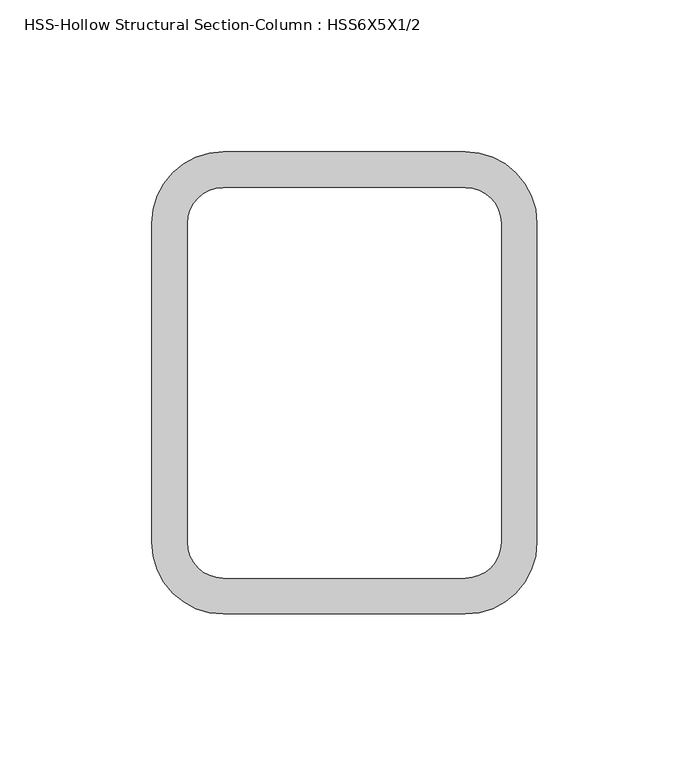
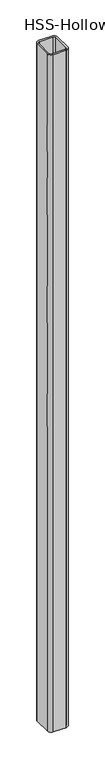
"""IFC4 building model written with IfcOpenShell, lengths in millimetres: column geometry, HSS-Hollow Structural Section-Column : HSS6X5X1/2."""

from ifc_helpers import new_model, si_unit, point, frame, frame_2d, origin, place, context, project, spatial, polyline, circle_curve, trimmed, segment, composite_curve, outline, extrude, source, transform, mapped, element, save


def hss_hollow_structural_section_column_hss6x5x1_2_cd1bbc2c(model_context):
    return source(origin(), model_context, "Body", "SweptSolid", [
        extrude(outline(composite_curve([segment(trimmed(circle_curve(frame_2d((39.878, 52.578)), 23.622), [point((39.878, 76.2))], [point((63.5, 52.578))], False, "CARTESIAN"), True, "CONTINUOUS"), segment(polyline([(63.5, 52.578), (63.5, -52.578)]), True, "CONTINUOUS"), segment(trimmed(circle_curve(frame_2d((39.878, -52.578)), 23.622), [point((63.5, -52.578))], [point((39.878, -76.2))], False, "CARTESIAN"), True, "CONTINUOUS"), segment(polyline([(39.878, -76.2), (-39.878, -76.2)]), True, "CONTINUOUS"), segment(trimmed(circle_curve(frame_2d((-39.878, -52.578)), 23.622), [point((-39.878, -76.2))], [point((-63.5, -52.578))], False, "CARTESIAN"), True, "CONTINUOUS"), segment(polyline([(-63.5, -52.578), (-63.5, 52.578)]), True, "CONTINUOUS"), segment(trimmed(circle_curve(frame_2d((-39.878, 52.578)), 23.622), [point((-63.5, 52.578))], [point((-39.878, 76.2))], False, "CARTESIAN"), True, "CONTINUOUS"), segment(polyline([(-39.878, 76.2), (39.878, 76.2)]), True, "CONTINUOUS")], self_intersect=False), holes=[composite_curve([segment(polyline([(39.878, 64.389), (-39.878, 64.389)]), True, "CONTINUOUS"), segment(trimmed(circle_curve(frame_2d((-39.878, 52.578)), 11.811), [point((-39.878, 64.389))], [point((-51.689, 52.578))], True, "CARTESIAN"), True, "CONTINUOUS"), segment(polyline([(-51.689, 52.578), (-51.689, -52.578)]), True, "CONTINUOUS"), segment(trimmed(circle_curve(frame_2d((-39.878, -52.578)), 11.811), [point((-51.689, -52.578))], [point((-39.878, -64.389))], True, "CARTESIAN"), True, "CONTINUOUS"), segment(polyline([(-39.878, -64.389), (39.878, -64.389)]), True, "CONTINUOUS"), segment(trimmed(circle_curve(frame_2d((39.878, -52.578)), 11.811), [point((39.878, -64.389))], [point((51.689, -52.578))], True, "CARTESIAN"), True, "CONTINUOUS"), segment(polyline([(51.689, -52.578), (51.689, 52.578)]), True, "CONTINUOUS"), segment(trimmed(circle_curve(frame_2d((39.878, 52.578)), 11.811), [point((51.689, 52.578))], [point((39.878, 64.389))], True, "CARTESIAN"), True, "CONTINUOUS")], self_intersect=False)]), frame((0.0, 0.0, -304.8), z_axis=(0.0, 0.0, 1.0), x_axis=(1.0, 0.0, 0.0)), (0.0, 0.0, 1.0), 4394.2),
    ])


if __name__ == "__main__":
    model = new_model("IFC4")
    model_context = context("Model", 3, world=origin())
    ifc_project = project(units=[si_unit("LENGTHUNIT", "METRE", prefix="MILLI")], contexts=[model_context])
    site = spatial("IfcSite", under=ifc_project)
    building = spatial("IfcBuilding", under=site)
    placement = place(None, origin())
    hss_hollow_structural_section_column_hss6x5x1_2_shape = hss_hollow_structural_section_column_hss6x5x1_2_cd1bbc2c(model_context)
    element("IfcColumn", 1, ObjectType="HSS-Hollow Structural Section-Column : HSS6X5X1/2", at=placement, inside=building, context=model_context, shape_type="MappedRepresentation", body=[
        mapped(hss_hollow_structural_section_column_hss6x5x1_2_shape, transform((0.0, 0.0, 0.0), x_axis=(1.0, 0.0, 0.0), y_axis=(0.0, 1.0, 0.0), z_axis=(0.0, 0.0, 1.0))),
    ])
    save(model, "model.ifc")

# Revit data of these elements
# Type "HSS-Hollow Structural Section-Column : HSS6X5X1/2"
#   Assembly Code = "B10"
#   Shape = "Rect."
#   W = 31.7
#   Ht = 0' - 6"
#   b = 0' - 5"
#   kr = 0' - 0.93"
#   t = 0' - 0.465"
#   A = 0.0611806 SF
#   Structural Material [instance default] = Steel ASTM A500, Grade B, Rectangular and Square
# Element 1 (IfcColumn, "HSS-Hollow Structural Section-Column : HSS6X5X1/2")
#   Structural Material = Metal - Steel - ASTM A992
#   Materials on its faces: "Metal - Steel - ASTM A992"
# Materials
#   "Steel ASTM A500, Grade B, Rectangular and Square": class "Metal", colour RGB 199 199 199, transparency 0, Description = "Carbon steel", Cost = 0
#   "Metal - Steel - ASTM A992": class "Metal", colour RGB 255 128 0, transparency 0
